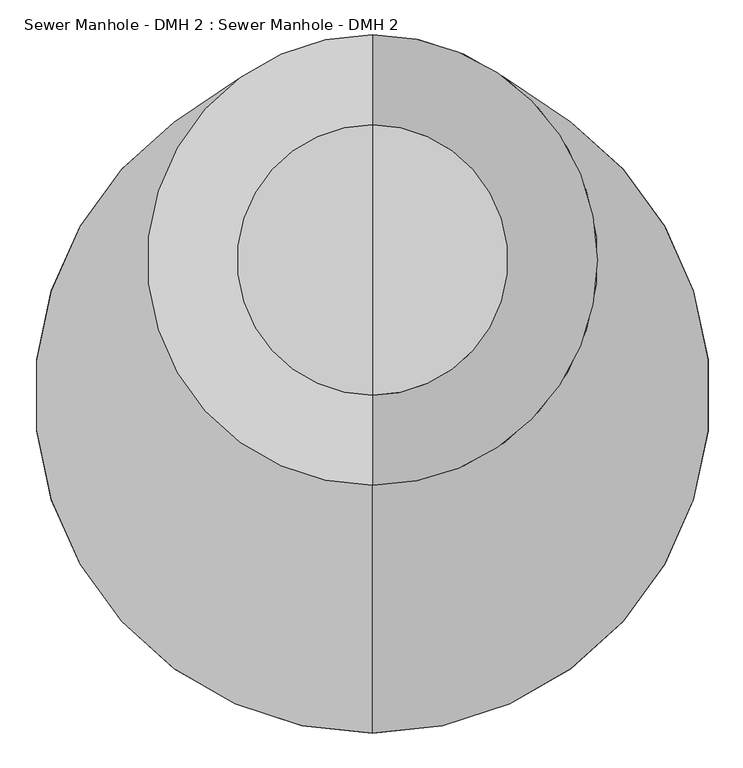
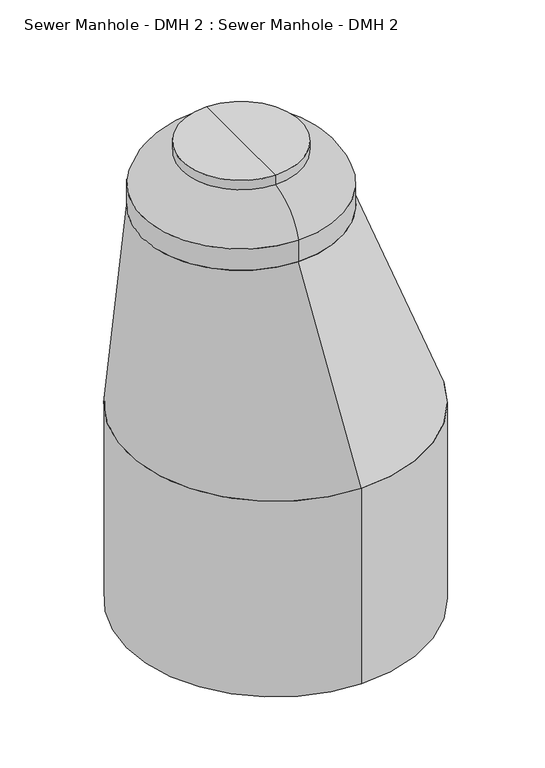
"""IFC4 building model written with IfcOpenShell, lengths in millimetres: proxy geometry, Sewer Manhole - DMH 2 : Sewer Manhole - DMH 2."""

from ifc_helpers import new_model, si_unit, point, frame, origin, place, context, project, spatial, circle_curve, ellipse_curve, trimmed, source, transform, mapped, element, save
from ifc_brep_helpers import plane_surface, cylinder_surface, revolved_surface, spline_surface, advanced_brep


def sewer_manhole_dmh_2_sewer_manhole_dmh_2_2724fa6c(model_context):
    return source(origin(), model_context, "Body", "AdvancedBrep", [
        advanced_brep(
        [(0.0, -203.2, 1942.3270774), (0.0, 812.8, 1942.3270774), (0.0, -762.0, 1056.64), (0.0, 762.0, 1056.64)],
        [
            (0, 1, circle_curve(frame((0.0, 304.8, 1942.3270774), z_axis=(0.0, 0.0, 1.0), x_axis=(0.0, 1.0, 0.0)), 508.0)),
            (1, 0, circle_curve(frame((0.0, 304.8, 1942.3270774), z_axis=(0.0, 0.0, 1.0), x_axis=(0.0, 1.0, 0.0)), 508.0)),
            (2, 3, circle_curve(frame((0.0, 0.0, 1056.64), z_axis=(0.0, 0.0, -1.0), x_axis=(0.0, 1.0, 0.0)), 762.0)),
            (3, 2, circle_curve(frame((0.0, 0.0, 1056.64), z_axis=(0.0, 0.0, -1.0), x_axis=(0.0, 1.0, 0.0)), 762.0)),
            (3, 1),
            (0, 2),
        ],
        [
            plane_surface(frame((0.0, 304.8, 1942.3270774), z_axis=(0.0, 0.0, 1.0), x_axis=(1.0, 0.0, 0.0))),
            plane_surface(frame((0.0, 0.0, 1056.64), z_axis=(0.0, 0.0, -1.0), x_axis=(1.0, 0.0, 0.0))),
            spline_surface(2, 1, [[(0.0, -762.0, 1056.64), (0.0, -203.2, 1942.3270774)], [(762.0, -762.0, 1056.64), (508.0, -203.2, 1942.3270774)], [(762.0, 0.0, 1056.64), (508.0, 304.8, 1942.3270774)], [(762.0, 762.0, 1056.64), (508.0, 812.8, 1942.3270774)], [(0.0, 762.0, 1056.64), (0.0, 812.8, 1942.3270774)]], [3, 2, 3], [2, 2], [0.0, 1.0, 2.0], [0.0, 1.0], weights=[[1.0, 1.0], [0.7071067811865476, 0.7071067811865476], [1.0, 1.0], [0.7071067811865476, 0.7071067811865476], [1.0, 1.0]]),
            spline_surface(2, 1, [[(0.0, 762.0, 1056.64), (0.0, 812.8, 1942.3270774)], [(-762.0, 762.0, 1056.64), (-507.99999999999994, 812.8, 1942.3270774)], [(-762.0, 0.0, 1056.64), (-507.99999999999994, 304.8, 1942.3270774)], [(-762.0, -762.0, 1056.64), (-507.99999999999994, -203.19999999999993, 1942.3270774)], [(0.0, -762.0, 1056.64), (0.0, -203.2, 1942.3270774)]], [3, 2, 3], [2, 2], [0.0, 1.0, 2.0], [0.0, 1.0], weights=[[1.0, 1.0], [0.7071067811865476, 0.7071067811865476], [1.0, 1.0], [0.7071067811865476, 0.7071067811865476], [1.0, 1.0]]),
        ],
        [
            (0, [[1, 2]]),
            (1, [[3, 4]]),
            (2, [[-4, 5, -1, 6]]),
            (3, [[-3, -6, -2, -5]]),
        ],
    ),
        advanced_brep(
        [(0.0, -203.2, 1942.3270774), (0.0, 812.8, 1942.3270774), (0.0, 304.8, 1942.3270774), (0.0, -203.2, 2057.4), (0.0, 812.8, 2057.4), (0.0, 0.0, 2235.2), (0.0, 609.6, 2235.2), (0.0, 0.0, 2286.0), (0.0, 609.6, 2286.0), (0.0, 304.8, 2286.0)],
        [
            (0, 1, circle_curve(frame((0.0, 304.8, 1942.3270774), z_axis=(0.0, 0.0, -1.0), x_axis=(0.0, 1.0, 0.0)), 508.0)),
            (1, 2),
            (2, 0),
            (1, 0, circle_curve(frame((0.0, 304.8, 1942.3270774), z_axis=(0.0, 0.0, -1.0), x_axis=(0.0, 1.0, 0.0)), 508.0)),
            (3, 4, circle_curve(frame((0.0, 304.8, 2057.4), z_axis=(0.0, 0.0, -1.0), x_axis=(0.0, 1.0, 0.0)), 508.0)),
            (4, 1),
            (0, 3),
            (4, 3, circle_curve(frame((0.0, 304.8, 2057.4), z_axis=(0.0, 0.0, -1.0), x_axis=(0.0, 1.0, 0.0)), 508.0)),
            (5, 6, circle_curve(frame((0.0, 304.8, 2235.2), z_axis=(0.0, 0.0, -1.0), x_axis=(0.0, 1.0, 0.0)), 304.8)),
            (6, 4, circle_curve(frame((0.0, 564.4539436, 1978.5902213), z_axis=(-1.0, 0.0, 0.0), x_axis=(0.0, -1.0, 0.0)), 260.550849)),
            (3, 5, circle_curve(frame((0.0, 45.1460564, 1978.5902213), z_axis=(-1.0, 0.0, 0.0), x_axis=(0.0, 1.0, 0.0)), 260.550849)),
            (6, 5, circle_curve(frame((0.0, 304.8, 2235.2), z_axis=(0.0, 0.0, -1.0), x_axis=(0.0, 1.0, 0.0)), 304.8)),
            (7, 8, circle_curve(frame((0.0, 304.8, 2286.0), z_axis=(0.0, 0.0, -1.0), x_axis=(0.0, 1.0, 0.0)), 304.8)),
            (8, 6),
            (5, 7),
            (8, 7, circle_curve(frame((0.0, 304.8, 2286.0), z_axis=(0.0, 0.0, -1.0), x_axis=(0.0, 1.0, 0.0)), 304.8)),
            (9, 8),
            (7, 9),
        ],
        [
            plane_surface(frame((0.0, 304.8, 1942.3270774), z_axis=(0.0, 0.0, -1.0), x_axis=(0.0, 1.0, 0.0))),
            cylinder_surface(frame((0.0, 304.8, 2006.6), z_axis=(0.0, 0.0, 1.0), x_axis=(0.0, 1.0, 0.0)), 508.0),
            revolved_surface(trimmed(ellipse_curve(frame((0.0, 564.4539436, 1978.5902213), z_axis=(1.0, 0.0, 0.0), x_axis=(0.0, -1.0, 0.0)), 260.550849, 260.550849), [point((0.0, 812.8, 2057.4))], [point((0.0, 609.6, 2235.2))], True, "CARTESIAN"), (0.0, 304.8, 2006.6), (0.0, 0.0, 1.0)),
            cylinder_surface(frame((0.0, 304.8, 2006.6), z_axis=(0.0, 0.0, 1.0), x_axis=(0.0, 1.0, 0.0)), 304.8),
            plane_surface(frame((0.0, 304.8, 2286.0), z_axis=(0.0, 0.0, 1.0), x_axis=(0.0, 1.0, 0.0))),
        ],
        [
            (0, [[1, 2, 3]]),
            (0, [[4, -3, -2]]),
            (1, [[5, 6, -1, 7]]),
            (1, [[8, -7, -4, -6]]),
            (2, [[9, 10, -5, 11]]),
            (2, [[12, -11, -8, -10]]),
            (3, [[13, 14, -9, 15]]),
            (3, [[16, -15, -12, -14]]),
            (4, [[17, -13, 18]]),
            (4, [[-18, -16, -17]]),
        ],
    ),
        advanced_brep(
        [(0.0, -762.0, 1056.64), (0.0, 762.0, 1056.64), (0.0, 762.0, 0.0), (0.0, -762.0, 0.0), (0.0, 0.0, 0.0), (0.0, 0.0, 1056.64)],
        [
            (0, 1, circle_curve(frame((0.0, 0.0, 1056.64), z_axis=(0.0, 0.0, -1.0), x_axis=(0.0, 1.0, 0.0)), 762.0)),
            (1, 2),
            (2, 3, circle_curve(frame((0.0, 0.0, 0.0), z_axis=(0.0, 0.0, 1.0), x_axis=(0.0, 1.0, 0.0)), 762.0)),
            (3, 0),
            (1, 0, circle_curve(frame((0.0, 0.0, 1056.64), z_axis=(0.0, 0.0, -1.0), x_axis=(0.0, 1.0, 0.0)), 762.0)),
            (3, 2, circle_curve(frame((0.0, 0.0, 0.0), z_axis=(0.0, 0.0, 1.0), x_axis=(0.0, 1.0, 0.0)), 762.0)),
            (2, 4),
            (4, 3),
            (5, 1),
            (0, 5),
        ],
        [
            cylinder_surface(frame((0.0, 0.0, 457.2), z_axis=(0.0, 0.0, 1.0), x_axis=(0.0, 1.0, 0.0)), 762.0),
            plane_surface(frame((0.0, 0.0, 0.0), z_axis=(0.0, 0.0, -1.0), x_axis=(0.0, 1.0, 0.0))),
            plane_surface(frame((0.0, 0.0, 1056.64), z_axis=(0.0, 0.0, 1.0), x_axis=(0.0, 1.0, 0.0))),
        ],
        [
            (0, [[1, 2, 3, 4]]),
            (0, [[5, -4, 6, -2]]),
            (1, [[-3, 7, 8]]),
            (1, [[-6, -8, -7]]),
            (2, [[9, -1, 10]]),
            (2, [[-10, -5, -9]]),
        ],
    ),
    ])


if __name__ == "__main__":
    model = new_model("IFC4")
    model_context = context("Model", 3, world=origin())
    ifc_project = project(units=[si_unit("LENGTHUNIT", "METRE", prefix="MILLI")], contexts=[model_context])
    site = spatial("IfcSite", under=ifc_project)
    building = spatial("IfcBuilding", under=site)
    placement = place(None, origin())
    sewer_manhole_dmh_2_sewer_manhole_dmh_2_shape = sewer_manhole_dmh_2_sewer_manhole_dmh_2_2724fa6c(model_context)
    element("IfcBuildingElementProxy", 1, Name="Sewer Manhole - DMH 2 : Sewer Manhole - DMH 2", ObjectType="Sewer Manhole - DMH 2 : Sewer Manhole - DMH 2", at=placement, inside=building, context=model_context, shape_type="MappedRepresentation", body=[
        mapped(sewer_manhole_dmh_2_sewer_manhole_dmh_2_shape, transform((0.0, 0.0, 0.0), x_axis=(1.0, 0.0, 0.0), y_axis=(0.0, 1.0, 0.0), z_axis=(0.0, 0.0, 1.0))),
    ])
    save(model, "model.ifc")
